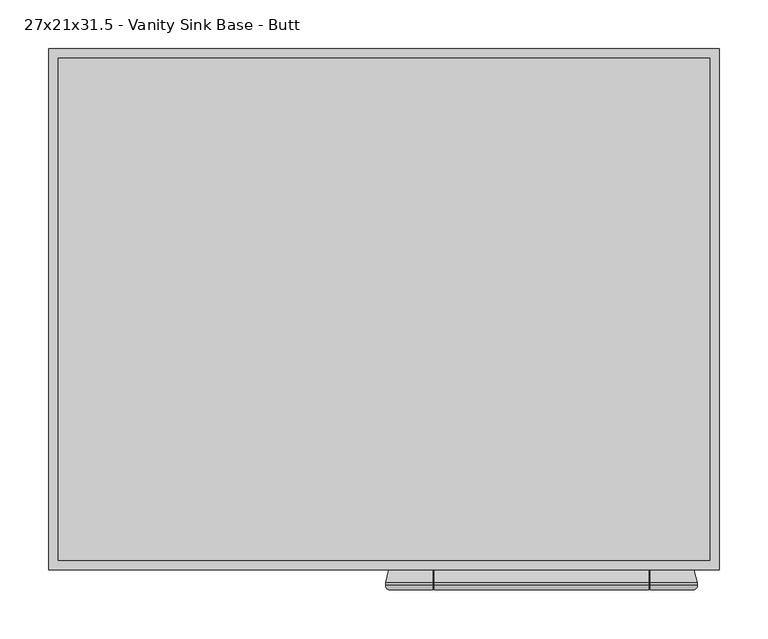
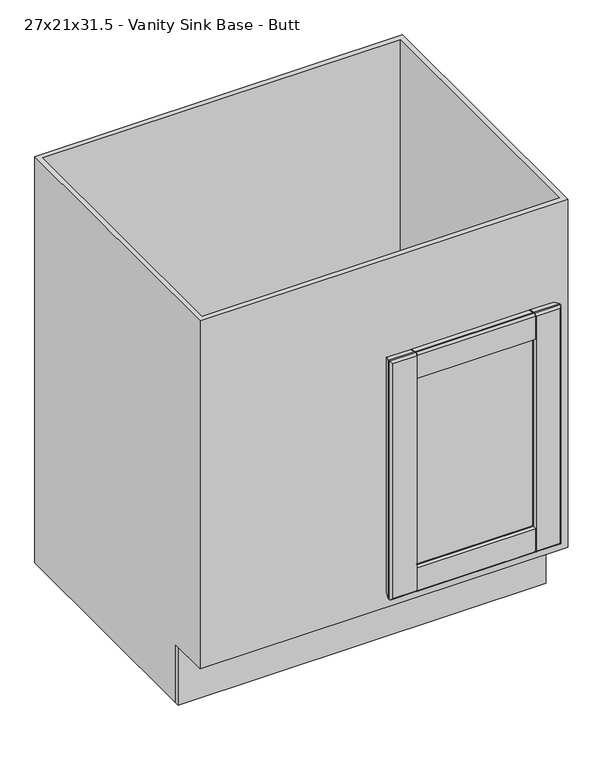
"""IFC4 building model written with IfcOpenShell, lengths in millimetres: furniture geometry, Cabinet-Base-Merillat-Double_Door-Marlin : 27x21x31.5 - Vanity Sink Base - Butt."""

from ifc_helpers import new_model, si_unit, frame, origin, origin_with_axes, place, context, project, spatial, polyline, circle_curve, ellipse_curve, outline, extrude, faceted_brep, source, transform, mapped, element, save
from ifc_brep_helpers import plane_surface, cylinder_surface, advanced_brep


def furniture_27x21x31_5_vanity_sink_base_butt_982747cf(model_context):
    return source(origin(), model_context, "Body", "SolidModel", [
        advanced_brep(
        [(339.4127049, -625.4496, 609.6), (336.3162124, -629.92, 606.5035075), (336.3162124, -629.92, 142.7964925), (339.4127049, -625.4496, 139.7), (339.4127049, -622.681, 139.7), (339.4127049, -622.681, 609.6), (335.9075049, -609.6, 143.2052), (335.9075049, -609.6, 606.0948), (291.2115422, -609.6, 561.3988372), (291.2115422, -609.6, 187.9011628), (290.8414105, -610.39375, 188.2712945), (288.7602514, -614.85681, 190.3524535), (288.7602514, -614.85681, 558.9475465), (290.8414105, -610.39375, 561.0287055), (290.1600209, -617.0969093, 188.952684), (290.1600209, -617.0969093, 560.347316), (304.4877049, -617.347, 174.625), (304.4877049, -617.347, 574.675), (304.4877049, -622.173, 174.625), (304.4877049, -622.173, 574.675), (290.1600209, -622.4230907, 188.952684), (290.1600209, -622.4230907, 560.347316), (288.7602514, -624.66319, 190.3524535), (288.7602514, -624.66319, 558.9475465), (290.8414105, -629.12625, 188.2712945), (291.2086747, -629.9138508, 187.9040302), (291.2115422, -629.92, 561.3988372), (290.8414105, -629.12625, 561.0287055), (291.2086747, -629.92, 142.7964925), (291.2086747, -625.4496, 139.7), (23.4216974, -629.92, 142.7964925), (20.3252049, -625.4496, 139.7), (68.4894236, -625.4496, 139.7), (68.4894236, -629.92, 142.7964925), (289.6211747, -625.4496, 139.7), (289.6211747, -629.92, 142.7964925), (70.0769236, -629.92, 142.7964925), (70.0769236, -625.4496, 139.7), (291.2086747, -622.681, 139.7), (20.3252049, -622.681, 139.7), (68.4894236, -622.681, 139.7), (289.6211747, -622.681, 139.7), (70.0769236, -622.681, 139.7), (291.2086747, -609.6, 143.2052), (23.8304049, -609.6, 143.2052), (68.4894236, -609.6, 143.2052), (289.6211747, -609.6, 143.2052), (70.0769236, -609.6, 143.2052), (70.9776584, -614.85681, 190.3524535), (289.6211747, -610.39375, 188.2712945), (289.6211747, -609.6, 187.9011628), (70.0769236, -609.6, 187.9011628), (70.0769236, -610.39375, 188.2712945), (68.8964994, -610.39375, 188.2712945), (69.577889, -617.0969093, 188.952684), (55.2502049, -617.347, 174.625), (55.2502049, -622.173, 174.625), (69.577889, -622.4230907, 188.952684), (70.9776584, -624.66319, 190.3524535), (68.8964994, -629.12625, 188.2712945), (70.0769236, -629.12625, 188.2712945), (70.0769236, -629.92, 187.9011628), (289.6211747, -629.92, 187.9011628), (289.6211747, -629.12625, 188.2712945), (23.4216974, -629.92, 606.5035075), (20.3252049, -625.4496, 609.6), (20.3252049, -622.681, 609.6), (23.8304049, -609.6, 606.0948), (68.5263677, -609.6, 187.9011628), (68.5263677, -609.6, 561.3988372), (68.8964994, -610.39375, 561.0287055), (70.9776584, -614.85681, 558.9475465), (69.577889, -617.0969093, 560.347316), (55.2502049, -617.347, 574.675), (55.2502049, -622.173, 574.675), (69.577889, -622.4230907, 560.347316), (70.9776584, -624.66319, 558.9475465), (68.8964994, -629.12625, 561.0287055), (68.5263677, -629.92, 561.3988372), (68.5263677, -629.92, 187.9011628), (68.4894236, -629.92, 606.5035075), (68.4894236, -625.4496, 609.6), (291.2086747, -625.4496, 609.6), (291.2086747, -629.92, 606.5035075), (70.0769236, -625.4496, 609.6), (70.0769236, -629.92, 606.5035075), (289.6211747, -629.92, 606.5035075), (289.6211747, -625.4496, 609.6), (68.4894236, -622.681, 609.6), (291.2086747, -622.681, 609.6), (70.0769236, -622.681, 609.6), (289.6211747, -622.681, 609.6), (68.4894236, -609.6, 606.0948), (291.2086747, -609.6, 606.0948), (70.0769236, -609.6, 606.0948), (289.6211747, -609.6, 606.0948), (70.0769236, -609.6, 561.3988372), (289.6211747, -609.6, 561.3988372), (70.0769236, -610.39375, 561.0287055), (289.6211747, -610.39375, 561.0287055), (289.6211747, -629.12625, 561.0287055), (289.6211747, -629.92, 561.3988372), (70.0769236, -629.92, 561.3988372), (70.0769236, -629.12625, 561.0287055), (70.0769236, -610.39375, 605.4857412), (70.0769236, -622.7855037, 608.80625), (70.0769236, -625.4496, 608.80625), (70.0769236, -629.12625, 606.3526052), (68.4894236, -629.12625, 561.0287055), (68.4894236, -629.12625, 606.3526052), (68.4894236, -625.4496, 608.80625), (68.4894236, -622.7855037, 608.80625), (68.4894236, -610.39375, 605.4857412), (68.4894236, -610.39375, 561.0287055), (291.2086747, -610.39375, 561.0287055), (291.2086747, -610.39375, 605.4857412), (291.2086747, -622.7855037, 608.80625), (291.2086747, -625.4496, 608.80625), (291.2086747, -629.12625, 606.3526052), (291.2086747, -629.12625, 561.0287055), (289.6211747, -629.12625, 606.3526052), (289.6211747, -625.4496, 608.80625), (289.6211747, -622.7855037, 608.80625), (289.6211747, -610.39375, 605.4857412), (291.2086747, -629.12625, 188.2712945), (291.2086747, -629.12625, 142.9473948), (291.2086747, -625.4496, 140.49375), (291.2086747, -622.7855037, 140.49375), (291.2086747, -610.39375, 143.8142588), (291.2086747, -610.39375, 188.2712945), (289.6211747, -610.39375, 143.8142588), (289.6211747, -622.7855037, 140.49375), (289.6211747, -625.4496, 140.49375), (289.6211747, -629.12625, 142.9473948), (70.0769236, -629.12625, 142.9473948), (70.0769236, -625.4496, 140.49375), (70.0769236, -622.7855037, 140.49375), (70.0769236, -610.39375, 143.8142588), (68.4894236, -629.12625, 188.2712945), (68.4894236, -610.39375, 188.2712945), (68.4894236, -610.39375, 143.8142588), (68.4894236, -622.7855037, 140.49375), (68.4894236, -625.4496, 140.49375), (68.4894236, -629.12625, 142.9473948)],
        [
            (0, 1, ellipse_curve(frame((334.6375049, -625.4496, 604.8248), z_axis=(0.7071067811865475, 0.0, -0.7071067811865475), x_axis=(0.7071067811865474, 0.0, 0.7071067811865476)), 6.7531526, 4.7752)),
            (1, 2),
            (2, 3, ellipse_curve(frame((334.6375049, -625.4496, 144.4752), z_axis=(0.7071067811865475, 0.0, 0.7071067811865475), x_axis=(-0.7071067811865474, 0.0, 0.7071067811865476)), 6.7531526, 4.7752)),
            (3, 0),
            (3, 4),
            (4, 5),
            (5, 0),
            (4, 6),
            (6, 7),
            (7, 5),
            (8, 9),
            (9, 10),
            (10, 11),
            (11, 12),
            (12, 13),
            (13, 8),
            (11, 14, ellipse_curve(frame((290.1875049, -615.5223492, 188.9252), z_axis=(0.7071067811865475, 0.0, 0.7071067811865475), x_axis=(-0.7071067811865474, 0.0, 0.7071067811865476)), 2.2271035, 1.5748)),
            (14, 15),
            (15, 12, ellipse_curve(frame((290.1875049, -615.5223492, 560.3748), z_axis=(0.7071067811865475, 0.0, -0.7071067811865475), x_axis=(0.7071067811865474, 0.0, 0.7071067811865476)), 2.2271035, 1.5748)),
            (14, 16),
            (16, 17),
            (17, 15),
            (16, 18),
            (18, 19),
            (19, 17),
            (18, 20),
            (20, 21),
            (21, 19),
            (20, 22, ellipse_curve(frame((290.1875049, -623.9976508, 188.9252), z_axis=(0.7071067811865475, 0.0, 0.7071067811865475), x_axis=(-0.7071067811865474, 0.0, 0.7071067811865476)), 2.2271035, 1.5748)),
            (22, 23),
            (23, 21, ellipse_curve(frame((290.1875049, -623.9976508, 560.3748), z_axis=(0.7071067811865475, 0.0, -0.7071067811865475), x_axis=(0.7071067811865474, 0.0, 0.7071067811865476)), 2.2271035, 1.5748)),
            (22, 24),
            (24, 25),
            (25, 26),
            (26, 27),
            (27, 23),
            (2, 28),
            (28, 29, circle_curve(frame((291.2086747, -625.4496, 144.4752), z_axis=(1.0, 0.0, 0.0), x_axis=(0.0, 1.0, 0.0)), 4.7752)),
            (29, 3),
            (30, 31, ellipse_curve(frame((25.1004049, -625.4496, 144.4752), z_axis=(0.7071067811865475, 0.0, -0.7071067811865475), x_axis=(0.7071067811865476, 0.0, 0.7071067811865474)), 6.7531526, 4.7752)),
            (31, 32),
            (32, 33, circle_curve(frame((68.4894236, -625.4496, 144.4752), z_axis=(-1.0, 0.0, 0.0), x_axis=(0.0, 1.0, 0.0)), 4.7752)),
            (33, 30),
            (34, 35, circle_curve(frame((289.6211747, -625.4496, 144.4752), z_axis=(-1.0, 0.0, 0.0), x_axis=(0.0, 1.0, 0.0)), 4.7752)),
            (35, 36),
            (36, 37, circle_curve(frame((70.0769236, -625.4496, 144.4752), z_axis=(1.0, 0.0, 0.0), x_axis=(0.0, 1.0, 0.0)), 4.7752)),
            (37, 34),
            (29, 38),
            (38, 4),
            (31, 39),
            (39, 40),
            (40, 32),
            (41, 34),
            (37, 42),
            (42, 41),
            (38, 43),
            (43, 6),
            (39, 44),
            (44, 45),
            (45, 40),
            (46, 41),
            (42, 47),
            (47, 46),
            (48, 11),
            (10, 49),
            (49, 50),
            (50, 51),
            (51, 52),
            (52, 53),
            (53, 48),
            (48, 54, ellipse_curve(frame((69.5504049, -615.5223492, 188.9252), z_axis=(0.7071067811865475, 0.0, -0.7071067811865475), x_axis=(0.7071067811865476, 0.0, 0.7071067811865474)), 2.2271035, 1.5748)),
            (54, 14),
            (54, 55),
            (55, 16),
            (55, 56),
            (56, 18),
            (56, 57),
            (57, 20),
            (57, 58, ellipse_curve(frame((69.5504049, -623.9976508, 188.9252), z_axis=(0.7071067811865475, 0.0, -0.7071067811865475), x_axis=(0.7071067811865476, 0.0, 0.7071067811865474)), 2.2271035, 1.5748)),
            (58, 22),
            (58, 59),
            (59, 60),
            (60, 61),
            (61, 62),
            (62, 63),
            (63, 24),
            (30, 64),
            (64, 65, ellipse_curve(frame((25.1004049, -625.4496, 604.8248), z_axis=(-0.7071067811865475, 0.0, -0.7071067811865475), x_axis=(0.7071067811865474, 0.0, -0.7071067811865476)), 6.7531526, 4.7752)),
            (65, 31),
            (65, 66),
            (66, 39),
            (66, 67),
            (67, 44),
            (68, 69),
            (69, 70),
            (70, 71),
            (71, 48),
            (53, 68),
            (71, 72, ellipse_curve(frame((69.5504049, -615.5223492, 560.3748), z_axis=(-0.7071067811865475, 0.0, -0.7071067811865475), x_axis=(0.7071067811865474, 0.0, -0.7071067811865476)), 2.2271035, 1.5748)),
            (72, 54),
            (72, 73),
            (73, 55),
            (73, 74),
            (74, 56),
            (74, 75),
            (75, 57),
            (75, 76, ellipse_curve(frame((69.5504049, -623.9976508, 560.3748), z_axis=(-0.7071067811865475, 0.0, -0.7071067811865475), x_axis=(0.7071067811865474, 0.0, -0.7071067811865476)), 2.2271035, 1.5748)),
            (76, 58),
            (76, 77),
            (77, 78),
            (78, 79),
            (79, 59),
            (64, 80),
            (80, 81, circle_curve(frame((68.4894236, -625.4496, 604.8248), z_axis=(-1.0, 0.0, 0.0), x_axis=(0.0, 1.0, 0.0)), 4.7752)),
            (81, 65),
            (0, 82),
            (82, 83, circle_curve(frame((291.2086747, -625.4496, 604.8248), z_axis=(1.0, 0.0, 0.0), x_axis=(0.0, 1.0, 0.0)), 4.7752)),
            (83, 1),
            (84, 85, circle_curve(frame((70.0769236, -625.4496, 604.8248), z_axis=(1.0, 0.0, 0.0), x_axis=(0.0, 1.0, 0.0)), 4.7752)),
            (85, 86),
            (86, 87, circle_curve(frame((289.6211747, -625.4496, 604.8248), z_axis=(-1.0, 0.0, 0.0), x_axis=(0.0, 1.0, 0.0)), 4.7752)),
            (87, 84),
            (81, 88),
            (88, 66),
            (5, 89),
            (89, 82),
            (90, 84),
            (87, 91),
            (91, 90),
            (88, 92),
            (92, 67),
            (7, 93),
            (93, 89),
            (94, 90),
            (91, 95),
            (95, 94),
            (43, 9),
            (8, 93),
            (92, 69),
            (68, 45),
            (96, 94),
            (95, 97),
            (97, 96),
            (50, 46),
            (47, 51),
            (12, 71),
            (70, 98),
            (98, 96),
            (97, 99),
            (99, 13),
            (15, 72),
            (17, 73),
            (19, 74),
            (21, 75),
            (23, 76),
            (27, 100),
            (100, 101),
            (101, 102),
            (102, 103),
            (103, 77),
            (83, 26),
            (25, 28),
            (33, 79),
            (78, 80),
            (85, 102),
            (101, 86),
            (35, 62),
            (61, 36),
            (98, 104),
            (104, 105),
            (105, 106),
            (106, 107, circle_curve(frame((70.0769236, -625.4496, 604.8248), z_axis=(1.0, 0.0, 0.0), x_axis=(0.0, 0.0, 1.0)), 3.98145)),
            (107, 103),
            (78, 108),
            (108, 109),
            (109, 110, circle_curve(frame((68.4894236, -625.4496, 604.8248), z_axis=(-1.0, 0.0, 0.0), x_axis=(0.0, 0.0, 1.0)), 3.98145)),
            (110, 111),
            (111, 112),
            (112, 113),
            (113, 69),
            (77, 108),
            (107, 109),
            (106, 110),
            (105, 111),
            (104, 112),
            (70, 113),
            (8, 114),
            (114, 115),
            (115, 116),
            (116, 117),
            (117, 118, circle_curve(frame((291.2086747, -625.4496, 604.8248), z_axis=(1.0, 0.0, 0.0), x_axis=(0.0, 0.0, 1.0)), 3.98145)),
            (118, 119),
            (119, 26),
            (100, 120),
            (120, 121, circle_curve(frame((289.6211747, -625.4496, 604.8248), z_axis=(-1.0, 0.0, 0.0), x_axis=(0.0, 0.0, 1.0)), 3.98145)),
            (121, 122),
            (122, 123),
            (123, 99),
            (119, 27),
            (118, 120),
            (117, 121),
            (116, 122),
            (115, 123),
            (114, 13),
            (25, 124),
            (124, 125),
            (125, 126, circle_curve(frame((291.2086747, -625.4496, 144.4752), z_axis=(1.0, 0.0, 0.0), x_axis=(0.0, 0.0, 1.0)), 3.98145)),
            (126, 127),
            (127, 128),
            (128, 129),
            (129, 9),
            (49, 130),
            (130, 131),
            (131, 132),
            (132, 133, circle_curve(frame((289.6211747, -625.4496, 144.4752), z_axis=(-1.0, 0.0, 0.0), x_axis=(0.0, 0.0, 1.0)), 3.98145)),
            (133, 63),
            (129, 10),
            (128, 130),
            (127, 131),
            (126, 132),
            (125, 133),
            (124, 24),
            (60, 134),
            (134, 135, circle_curve(frame((70.0769236, -625.4496, 144.4752), z_axis=(1.0, 0.0, 0.0), x_axis=(0.0, 0.0, 1.0)), 3.98145)),
            (135, 136),
            (136, 137),
            (137, 52),
            (138, 79),
            (68, 139),
            (139, 140),
            (140, 141),
            (141, 142),
            (142, 143, circle_curve(frame((68.4894236, -625.4496, 144.4752), z_axis=(-1.0, 0.0, 0.0), x_axis=(0.0, 0.0, 1.0)), 3.98145)),
            (143, 138),
            (138, 59),
            (53, 139),
            (137, 140),
            (136, 141),
            (135, 142),
            (134, 143),
        ],
        [
            cylinder_surface(frame((334.6375049, -625.4496, 609.6), z_axis=(0.0, 0.0, 1.0), x_axis=(0.0, 1.0, 0.0)), 4.7752),
            plane_surface(frame((339.4127049, -625.4496, 609.6), z_axis=(1.0, 0.0, 0.0), x_axis=(0.0, 0.0, -1.0))),
            plane_surface(frame((339.4127049, -622.681, 609.6), z_axis=(0.9659229350723619, 0.25882983502910506, 0.0), x_axis=(0.0, 0.0, -1.0))),
            plane_surface(frame((291.2115422, -609.6, 561.3988372), z_axis=(-0.9063077870366099, 0.4226182617407856, 0.0), x_axis=(0.0, 0.0, -1.0))),
            cylinder_surface(frame((290.1875049, -615.5223492, 609.6), z_axis=(0.0, 0.0, 1.0000000000000002), x_axis=(-0.01745240643729364, -0.9998476951563912, 0.0)), 1.5748),
            plane_surface(frame((290.1600209, -617.0969093, 560.347316), z_axis=(-0.017452406437322144, -0.9998476951563906, 0.0), x_axis=(0.0, 0.0, -1.0))),
            plane_surface(frame((304.4877049, -617.347, 574.675), z_axis=(-1.0, 0.0, 0.0), x_axis=(0.0, 0.0, -1.0))),
            plane_surface(frame((304.4877049, -622.173, 574.675), z_axis=(-0.01745240643727848, 0.9998476951563914, 0.0), x_axis=(0.0, 0.0, -1.0))),
            cylinder_surface(frame((290.1875049, -623.9976508, 609.6), z_axis=(0.0, 0.0, 1.0000000000000002), x_axis=(-0.9063077870367326, -0.42261826174052236, 0.0)), 1.5748),
            plane_surface(frame((288.7602514, -624.66319, 558.9475465), z_axis=(-0.9063077870366333, -0.4226182617407352, 0.0), x_axis=(0.0, 0.0, -1.0))),
            cylinder_surface(frame((339.4127049, -625.4496, 144.4752), z_axis=(1.0, 0.0, 0.0), x_axis=(0.0, 1.0, 0.0)), 4.7752),
            plane_surface(frame((339.4127049, -625.4496, 139.7), z_axis=(0.0, 0.0, -1.0), x_axis=(-1.0, 0.0, 0.0))),
            plane_surface(frame((339.4127049, -622.681, 139.7), z_axis=(0.0, 0.25882983502910506, -0.9659229350723619), x_axis=(-1.0, 0.0, 0.0))),
            plane_surface(frame((291.2115422, -609.6, 187.9011628), z_axis=(0.0, 0.4226182617407856, 0.9063077870366099), x_axis=(-1.0, 0.0, 0.0))),
            cylinder_surface(frame((339.4127049, -615.5223492, 188.9252), z_axis=(1.0000000000000002, 0.0, 0.0), x_axis=(0.0, -0.9998476951563912, 0.01745240643729364)), 1.5748),
            plane_surface(frame((290.1600209, -617.0969093, 188.952684), z_axis=(0.0, -0.9998476951563906, 0.017452406437322144), x_axis=(-1.0, 0.0, 0.0))),
            plane_surface(frame((304.4877049, -617.347, 174.625), z_axis=(0.0, 0.0, 1.0), x_axis=(-1.0, 0.0, 0.0))),
            plane_surface(frame((304.4877049, -622.173, 174.625), z_axis=(0.0, 0.9998476951563914, 0.01745240643727848), x_axis=(-1.0, 0.0, 0.0))),
            cylinder_surface(frame((339.4127049, -623.9976508, 188.9252), z_axis=(1.0000000000000002, 0.0, 0.0), x_axis=(0.0, -0.42261826174052236, 0.9063077870367326)), 1.5748),
            plane_surface(frame((288.7602514, -624.66319, 190.3524535), z_axis=(0.0, -0.4226182617407352, 0.9063077870366333), x_axis=(-1.0, 0.0, 0.0))),
            cylinder_surface(frame((25.1004049, -625.4496, 139.7), z_axis=(0.0, 0.0, -1.0), x_axis=(0.0, 1.0, 0.0)), 4.7752),
            plane_surface(frame((20.3252049, -625.4496, 139.7), z_axis=(-1.0, 0.0, 0.0), x_axis=(0.0, 0.0, 1.0))),
            plane_surface(frame((20.3252049, -622.681, 139.7), z_axis=(-0.9659229350723619, 0.25882983502910506, 0.0), x_axis=(0.0, 0.0, 1.0))),
            plane_surface(frame((68.5263677, -609.6, 187.9011628), z_axis=(0.9063077870366099, 0.4226182617407856, 0.0), x_axis=(0.0, 0.0, 1.0))),
            cylinder_surface(frame((69.5504049, -615.5223492, 139.7), z_axis=(0.0, 0.0, -1.0000000000000002), x_axis=(0.01745240643729364, -0.9998476951563912, 0.0)), 1.5748),
            plane_surface(frame((69.577889, -617.0969093, 188.952684), z_axis=(0.017452406437322144, -0.9998476951563906, 0.0), x_axis=(0.0, 0.0, 1.0))),
            plane_surface(frame((55.2502049, -617.347, 174.625), z_axis=(1.0, 0.0, 0.0), x_axis=(0.0, 0.0, 1.0))),
            plane_surface(frame((55.2502049, -622.173, 174.625), z_axis=(0.01745240643727848, 0.9998476951563914, 0.0), x_axis=(0.0, 0.0, 1.0))),
            cylinder_surface(frame((69.5504049, -623.9976508, 139.7), z_axis=(0.0, 0.0, -1.0000000000000002), x_axis=(0.9063077870367326, -0.42261826174052236, 0.0)), 1.5748),
            plane_surface(frame((70.9776584, -624.66319, 190.3524535), z_axis=(0.9063077870366333, -0.4226182617407352, 0.0), x_axis=(0.0, 0.0, 1.0))),
            cylinder_surface(frame((20.3252049, -625.4496, 604.8248), z_axis=(-1.0, 0.0, 0.0), x_axis=(0.0, 1.0, 0.0)), 4.7752),
            plane_surface(frame((20.3252049, -625.4496, 609.6), z_axis=(0.0, 0.0, 1.0), x_axis=(1.0, 0.0, 0.0))),
            plane_surface(frame((20.3252049, -622.681, 609.6), z_axis=(0.0, 0.25882983502910506, 0.9659229350723619), x_axis=(1.0, 0.0, 0.0))),
            plane_surface(frame((23.8304049, -609.6, 606.0948), z_axis=(0.0, 1.0, 0.0), x_axis=(1.0, 0.0, 0.0))),
            plane_surface(frame((68.5263677, -609.6, 561.3988372), z_axis=(0.0, 0.4226182617407856, -0.9063077870366099), x_axis=(1.0, 0.0, 0.0))),
            cylinder_surface(frame((20.3252049, -615.5223492, 560.3748), z_axis=(-1.0000000000000002, 0.0, 0.0), x_axis=(0.0, -0.9998476951563912, -0.01745240643729364)), 1.5748),
            plane_surface(frame((69.577889, -617.0969093, 560.347316), z_axis=(0.0, -0.9998476951563906, -0.017452406437322144), x_axis=(1.0, 0.0, 0.0))),
            plane_surface(frame((55.2502049, -617.347, 574.675), z_axis=(0.0, 0.0, -1.0), x_axis=(1.0, 0.0, 0.0))),
            plane_surface(frame((55.2502049, -622.173, 574.675), z_axis=(0.0, 0.9998476951563914, -0.01745240643727848), x_axis=(1.0, 0.0, 0.0))),
            cylinder_surface(frame((20.3252049, -623.9976508, 560.3748), z_axis=(-1.0000000000000002, 0.0, 0.0), x_axis=(0.0, -0.42261826174052236, -0.9063077870367326)), 1.5748),
            plane_surface(frame((70.9776584, -624.66319, 558.9475465), z_axis=(0.0, -0.4226182617407352, -0.9063077870366333), x_axis=(1.0, 0.0, 0.0))),
            plane_surface(frame((68.5263677, -629.92, 561.3988372), z_axis=(0.0, -1.0, 0.0), x_axis=(1.0, 0.0, 0.0))),
            plane_surface(frame((70.0769236, -629.92, 561.3988372), z_axis=(-1.0, 0.0, 0.0), x_axis=(0.0, 0.9063077870366341, -0.4226182617407336))),
            plane_surface(frame((68.4894236, -629.92, 561.3988372), z_axis=(1.0, 0.0, 0.0), x_axis=(0.0, -0.9063077870366341, 0.4226182617407336))),
            plane_surface(frame((70.0769236, -629.92, 561.3988372), z_axis=(0.0, 0.4226182617407336, 0.9063077870366341), x_axis=(-1.0, 0.0, 0.0))),
            plane_surface(frame((70.0769236, -629.12625, 561.0287055), z_axis=(0.0, -1.0, 0.0), x_axis=(-1.0, 0.0, 0.0))),
            cylinder_surface(frame((68.4894236, -625.4496, 604.8248), z_axis=(-1.0, 0.0, 0.0), x_axis=(0.0, 0.0, 1.0)), 3.98145),
            plane_surface(frame((70.0769236, -625.4496, 608.80625), z_axis=(0.0, 0.0, 1.0), x_axis=(-1.0, 0.0, 0.0))),
            plane_surface(frame((70.0769236, -622.7855037, 608.80625), z_axis=(0.0, 0.2588298350291669, 0.9659229350723454), x_axis=(-1.0, 0.0, 0.0))),
            plane_surface(frame((70.0769236, -610.39375, 605.4857412), z_axis=(0.0, 1.0, 0.0), x_axis=(-1.0, 0.0, 0.0))),
            plane_surface(frame((70.0769236, -610.39375, 561.0287055), z_axis=(0.0, -0.42261826174081096, 0.906307787036598), x_axis=(-1.0, 0.0, 0.0))),
            plane_surface(frame((291.2086747, -629.92, 561.3988372), z_axis=(-1.0000000000000002, 0.0, 0.0), x_axis=(0.0, 0.9063077870366427, -0.42261826174071515))),
            plane_surface(frame((289.6211747, -629.92, 561.3988372), z_axis=(1.0000000000000002, 0.0, 0.0), x_axis=(0.0, -0.9063077870366427, 0.42261826174071515))),
            plane_surface(frame((291.2086747, -629.92, 561.3988372), z_axis=(0.0, 0.42261826174071515, 0.9063077870366427), x_axis=(-1.0, 0.0, 0.0))),
            plane_surface(frame((291.2086747, -629.12625, 561.0287055), z_axis=(0.0, -1.0, 0.0), x_axis=(-1.0, 0.0, 0.0))),
            cylinder_surface(frame((289.6211747, -625.4496, 604.8248), z_axis=(-1.0, 0.0, 0.0), x_axis=(0.0, 0.0, 1.0)), 3.98145),
            plane_surface(frame((291.2086747, -625.4496, 608.80625), z_axis=(0.0, 0.0, 1.0), x_axis=(-1.0, 0.0, 0.0))),
            plane_surface(frame((291.2086747, -622.7855037, 608.80625), z_axis=(0.0, 0.25882983502916707, 0.9659229350723454), x_axis=(-1.0, 0.0, 0.0))),
            plane_surface(frame((291.2086747, -610.39375, 605.4857412), z_axis=(0.0, 1.0, 0.0), x_axis=(-1.0, 0.0, 0.0))),
            plane_surface(frame((291.2086747, -610.39375, 561.0287055), z_axis=(0.0, -0.42261826174082806, 0.9063077870365901), x_axis=(-1.0, 0.0, 0.0))),
            plane_surface(frame((291.2086747, -625.4496, 149.2504), z_axis=(-1.0, 0.0, 0.0), x_axis=(0.0, -1.0, 0.0))),
            plane_surface(frame((289.6211747, -625.4496, 149.2504), z_axis=(1.0, 0.0, 0.0), x_axis=(0.0, 1.0, 0.0))),
            plane_surface(frame((291.2086747, -609.6, 187.9011628), z_axis=(0.0, -0.4226182617407918, -0.906307787036607), x_axis=(-1.0, 0.0, 0.0))),
            plane_surface(frame((291.2086747, -610.39375, 188.2712945), z_axis=(0.0, 1.0, 0.0), x_axis=(-1.0, 0.0, 0.0))),
            plane_surface(frame((291.2086747, -610.39375, 143.8142588), z_axis=(0.0, 0.25882983502943513, -0.9659229350722734), x_axis=(-1.0, 0.0, 0.0))),
            plane_surface(frame((291.2086747, -622.7855037, 140.49375), z_axis=(0.0, 0.0, -1.0), x_axis=(-1.0, 0.0, 0.0))),
            cylinder_surface(frame((289.6211747, -625.4496, 144.4752), z_axis=(-1.0, 0.0, 0.0), x_axis=(0.0, 0.0, 1.0)), 3.98145),
            plane_surface(frame((291.2086747, -629.12625, 142.9473948), z_axis=(0.0, -1.0, 0.0), x_axis=(-1.0, 0.0, 0.0))),
            plane_surface(frame((291.2086747, -629.12625, 188.2712945), z_axis=(0.0, 0.42261826174073647, -0.9063077870366327), x_axis=(-1.0, 0.0, 0.0))),
            plane_surface(frame((70.0769236, -629.12625, 188.2712945), z_axis=(-1.0, 0.0, 0.0), x_axis=(0.0, -0.9063077870366302, -0.42261826174074196))),
            plane_surface(frame((68.4894236, -629.12625, 188.2712945), z_axis=(1.0, 0.0, 0.0), x_axis=(0.0, 0.9063077870366302, 0.42261826174074196))),
            plane_surface(frame((70.0769236, -629.12625, 188.2712945), z_axis=(0.0, 0.42261826174074196, -0.9063077870366302), x_axis=(-1.0, 0.0, 0.0))),
            plane_surface(frame((70.0769236, -609.6, 187.9011628), z_axis=(0.0, -0.4226182617408051, -0.9063077870366008), x_axis=(-1.0, 0.0, 0.0))),
            plane_surface(frame((70.0769236, -610.39375, 188.2712945), z_axis=(0.0, 1.0, 0.0), x_axis=(-1.0, 0.0, 0.0))),
            plane_surface(frame((70.0769236, -610.39375, 143.8142588), z_axis=(0.0, 0.258829835029436, -0.9659229350722733), x_axis=(-1.0, 0.0, 0.0))),
            plane_surface(frame((70.0769236, -622.7855037, 140.49375), z_axis=(0.0, 0.0, -1.0), x_axis=(-1.0, 0.0, 0.0))),
            cylinder_surface(frame((68.4894236, -625.4496, 144.4752), z_axis=(-1.0, 0.0, 0.0), x_axis=(0.0, 0.0, 1.0)), 3.98145),
            plane_surface(frame((70.0769236, -629.12625, 142.9473948), z_axis=(0.0, -1.0, 0.0), x_axis=(-1.0, 0.0, 0.0))),
        ],
        [
            (0, [[1, 2, 3, 4]]),
            (1, [[-4, 5, 6, 7]]),
            (2, [[-6, 8, 9, 10]]),
            (3, [[11, 12, 13, 14, 15, 16]]),
            (4, [[-14, 17, 18, 19]]),
            (5, [[-18, 20, 21, 22]]),
            (6, [[-21, 23, 24, 25]]),
            (7, [[-24, 26, 27, 28]]),
            (8, [[-27, 29, 30, 31]]),
            (9, [[-30, 32, 33, 34, 35, 36]]),
            (10, [[-3, 37, 38, 39]]),
            (10, [[40, 41, 42, 43]]),
            (10, [[44, 45, 46, 47]]),
            (11, [[-5, -39, 48, 49]]),
            (11, [[50, 51, 52, -41]]),
            (11, [[53, -47, 54, 55]]),
            (12, [[-8, -49, 56, 57]]),
            (12, [[58, 59, 60, -51]]),
            (12, [[61, -55, 62, 63]]),
            (13, [[64, -13, 65, 66, 67, 68, 69, 70]]),
            (14, [[-17, -64, 71, 72]]),
            (15, [[-20, -72, 73, 74]]),
            (16, [[-23, -74, 75, 76]]),
            (17, [[-26, -76, 77, 78]]),
            (18, [[-29, -78, 79, 80]]),
            (19, [[-80, 81, 82, 83, 84, 85, 86, -32]]),
            (20, [[-40, 87, 88, 89]]),
            (21, [[-50, -89, 90, 91]]),
            (22, [[-58, -91, 92, 93]]),
            (23, [[94, 95, 96, 97, -70, 98]]),
            (24, [[-71, -97, 99, 100]]),
            (25, [[-73, -100, 101, 102]]),
            (26, [[-75, -102, 103, 104]]),
            (27, [[-77, -104, 105, 106]]),
            (28, [[-79, -106, 107, 108]]),
            (29, [[-108, 109, 110, 111, 112, -81]]),
            (30, [[-88, 113, 114, 115]]),
            (30, [[-1, 116, 117, 118]]),
            (30, [[119, 120, 121, 122]]),
            (31, [[-90, -115, 123, 124]]),
            (31, [[-7, 125, 126, -116]]),
            (31, [[127, -122, 128, 129]]),
            (32, [[-92, -124, 130, 131]]),
            (32, [[-10, 132, 133, -125]]),
            (32, [[134, -129, 135, 136]]),
            (33, [[-9, -57, 137, -11, 138, -132]]),
            (33, [[-93, -131, 139, -94, 140, -59]]),
            (33, [[141, -136, 142, 143]]),
            (33, [[144, -63, 145, -67]]),
            (34, [[146, -96, 147, 148, -143, 149, 150, -15]]),
            (35, [[-19, 151, -99, -146]]),
            (36, [[-22, 152, -101, -151]]),
            (37, [[-25, 153, -103, -152]]),
            (38, [[-28, 154, -105, -153]]),
            (39, [[-31, 155, -107, -154]]),
            (40, [[-155, -36, 156, 157, 158, 159, 160, -109]]),
            (41, [[-2, -118, 161, -34, 162, -37]]),
            (41, [[-87, -43, 163, -111, 164, -113]]),
            (41, [[165, -158, 166, -120]]),
            (41, [[167, -84, 168, -45]]),
            (42, [[169, 170, 171, 172, 173, -159, -165, -119, -127, -134, -141, -148]]),
            (43, [[174, 175, 176, 177, 178, 179, 180, -139, -130, -123, -114, -164]]),
            (44, [[-174, -110, 181]]),
            (45, [[-173, 182, -175, -181, -160]]),
            (46, [[-172, 183, -176, -182]]),
            (47, [[-171, 184, -177, -183]]),
            (48, [[-170, 185, -178, -184]]),
            (49, [[-169, -147, 186, -179, -185]]),
            (50, [[-180, -186, -95]]),
            (51, [[187, 188, 189, 190, 191, 192, 193, -161, -117, -126, -133, -138]]),
            (52, [[194, 195, 196, 197, 198, -149, -142, -135, -128, -121, -166, -157]]),
            (53, [[-193, 199, -35]]),
            (54, [[-192, 200, -194, -156, -199]]),
            (55, [[-191, 201, -195, -200]]),
            (56, [[-190, 202, -196, -201]]),
            (57, [[-189, 203, -197, -202]]),
            (58, [[-188, 204, -150, -198, -203]]),
            (59, [[-187, -16, -204]]),
            (60, [[205, 206, 207, 208, 209, 210, 211, -137, -56, -48, -38, -162]]),
            (61, [[212, 213, 214, 215, 216, -85, -167, -44, -53, -61, -144, -66]]),
            (62, [[-211, 217, -12]]),
            (63, [[-210, 218, -212, -65, -217]]),
            (64, [[-209, 219, -213, -218]]),
            (65, [[-208, 220, -214, -219]]),
            (66, [[-207, 221, -215, -220]]),
            (67, [[-206, 222, -86, -216, -221]]),
            (68, [[-205, -33, -222]]),
            (69, [[223, 224, 225, 226, 227, -68, -145, -62, -54, -46, -168, -83]]),
            (70, [[228, -163, -42, -52, -60, -140, 229, 230, 231, 232, 233, 234]]),
            (71, [[-228, 235, -112]]),
            (72, [[-229, -98, 236]]),
            (73, [[-227, 237, -230, -236, -69]]),
            (74, [[-226, 238, -231, -237]]),
            (75, [[-225, 239, -232, -238]]),
            (76, [[-224, 240, -233, -239]]),
            (77, [[-223, -82, -235, -234, -240]]),
        ],
    ),
        extrude(outline(polyline([(55.2502049, -622.173), (55.2502049, -617.347), (304.4877049, -617.347), (304.4877049, -622.173), (55.2502049, -622.173)])), frame((0.0, 0.0, 174.625), z_axis=(0.0, 0.0, 1.0), x_axis=(1.0, 0.0, 0.0)), (0.0, 0.0, 1.0), 400.05),
        faceted_brep([(361.6377049, -76.2, 0.0), (361.6377049, -529.43125, 0.0), (352.1127049, -529.43125, 0.0), (352.1127049, -85.725, 0.0), (-314.6372951, -85.725, 0.0), (-314.6372951, -529.43125, 0.0), (-324.1622951, -529.43125, 0.0), (-324.1622951, -76.2, 0.0), (-324.1622951, -76.2, 800.1), (361.6377049, -76.2, 800.1), (-324.1622951, -529.43125, 114.3), (-324.1622951, -609.6, 114.3), (-324.1622951, -609.6, 800.1), (361.6377049, -609.6, 800.1), (361.6377049, -609.6, 114.3), (361.6377049, -529.43125, 114.3), (352.1127049, -529.43125, 114.3), (352.1127049, -85.725, 114.3), (352.1127049, -600.075, 800.1), (352.1127049, -85.725, 800.1), (352.1127049, -85.725, 123.825), (352.1127049, -600.075, 123.825), (-314.6372951, -85.725, 114.3), (-314.6372951, -529.43125, 114.3), (-314.6372951, -85.725, 800.1), (-314.6372951, -600.075, 800.1), (-314.6372951, -600.075, 123.825), (-314.6372951, -85.725, 123.825)], [[[0, 1, 2, 3, 4, 5, 6, 7]], [[0, 7, 8, 9]], [[7, 6, 10, 11, 12, 8]], [[1, 0, 9, 13, 14, 15]], [[3, 2, 16, 17]], [[18, 19, 20, 21]], [[5, 4, 22, 23]], [[24, 25, 26, 27]], [[4, 3, 17, 22]], [[19, 24, 27, 20]], [[9, 8, 12, 13], [19, 18, 25, 24]], [[14, 11, 10, 23, 22, 17, 16, 15]], [[13, 12, 11, 14]], [[25, 18, 21, 26]], [[6, 5, 23, 10]], [[2, 1, 15, 16]], [[21, 20, 27, 26]]]),
        extrude(outline(polyline([(361.6377049, -529.43125), (361.6377049, -538.95625), (-324.1622951, -538.95625), (-324.1622951, -529.43125), (361.6377049, -529.43125)])), origin_with_axes(), (0.0, 0.0, 1.0), 114.3),
    ])


if __name__ == "__main__":
    model = new_model("IFC4")
    model_context = context("Model", 3, world=origin())
    ifc_project = project(units=[si_unit("LENGTHUNIT", "METRE", prefix="MILLI")], contexts=[model_context])
    site = spatial("IfcSite", under=ifc_project)
    building = spatial("IfcBuilding", under=site)
    placement = place(None, origin())
    furniture_27x21x31_5_vanity_sink_base_butt_shape = furniture_27x21x31_5_vanity_sink_base_butt_982747cf(model_context)
    element("IfcFurniture", 1, ObjectType="Cabinet-Base-Merillat-Double_Door-Marlin : 27x21x31.5 - Vanity Sink Base - Butt", at=placement, inside=building, context=model_context, shape_type="MappedRepresentation", body=[
        mapped(furniture_27x21x31_5_vanity_sink_base_butt_shape, transform((0.0, 0.0, 0.0), x_axis=(1.0, 0.0, 0.0), y_axis=(0.0, 1.0, 0.0), z_axis=(0.0, 0.0, 1.0))),
    ])
    save(model, "model.ifc")

# Revit data of these elements
# Type "Cabinet-Base-Merillat-Double_Door-Marlin : 27x21x31.5 - Vanity Sink Base - Butt"
#   URL = "http://www.merillat.com"
#   Toe Kick Note = "Toe Kick Covering is not included. To be purchased Separately."
#   Product Line = "Express"
#   Product Page URL = "http://www.merillat.com//our-products/rooms/bathroom"
#   Product Group = "Vanity Cabinet"
#   Product Documentation Link = "http://merillatbusiness.com/customer-resources/product-line-resources/merillat-classic/"
#   Model = "VSB30B"
#   Manufacturer = "Merillat"
#   Finish = "Wood"
#   Description = "Vanity Sink Base Butt Door"
#   Construction Type = "Deep Sink Base"
#   Cabinet Construction Note = "No shelf, cabinets w/ a \"B\" suffix have BUTT doors without a center frame stile,  VSB39, VSB42. VSB3935 and VSB4235 have a double door with a frame center stile, All cabinets have one full-width drawer front except VSB42 and VSB4235 which have two drawer fronts"
#   Assembly Code = "C1030410"
#   Toe Kick Height = 0' - 4 1/2"
#   Toe Kick Depth = 0' - 2 25/32"
#   Top and Bottom Spacing = 0' - 1"
#   Side Spacing = 0' - 0 7/8"
#   Cabinet Shell = 0' - 0 3/8"
#   Door Spacing = 0' - 0 1/8"
#   Depth = 1' - 9"
#   Height = 2' - 7 1/2"
#   Width = 2' - 3"
#   Cabinet Drawer Width = 2' - 1 1/4"
#   Cabinet Drawer Height = 0' - 5 1/2"
#   Cabinet Drawer 2 Drawer Width = 1' - 0 9/16"
#   Cabinet Door Width = 1' - 0 9/16"
#   Cabinet Door Height = 1' - 6 1/2"
#   COBie.Type = no
#   Two Drawer = no
#   Elevation Swing Line = yes
#   Partial Overlay = yes
#   One Drawer = yes
#   Full Overlay = no
#   Butt Option = yes
#   Toe Kick Material = Wood - Merillat - Raw Particle Board
#   Door Drawer Material = Wood - Merillat - Pecan(1)
#   Cabinet Material = Wood - Merillat - Pecan(1)
#   Cabinet Drawer Style 2 Drawer = element 819256
#   Cabinet Drawer Style = element 819255
#   Cabinet Door Style = element 819254
# Element 1 (IfcFurniture, "Cabinet-Base-Merillat-Double_Door-Marlin : 27x21x31.5 - Vanity Sink Base - Butt")
#   Materials on its faces: "Wood - Merillat - Pecan(1)", "Wood - Merillat - Raw Particle Board"
# Materials
#   "Wood - Merillat - Raw Particle Board": class "Plastic", colour RGB 80 80 80, transparency 0, Description = "Plastic Laminate - Navy", Cost = 0
#   "Wood - Merillat - Pecan(1)": class "Wood", colour RGB 108 67 43, transparency 0, Cost = 0
